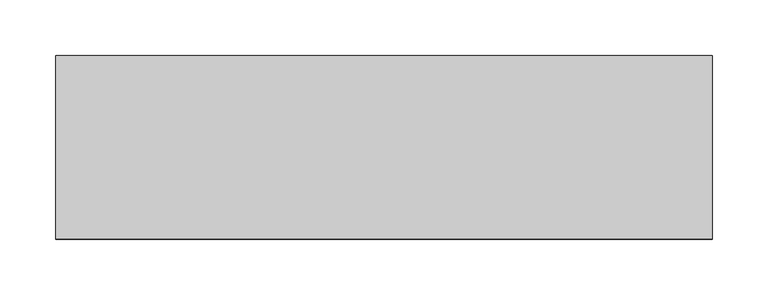
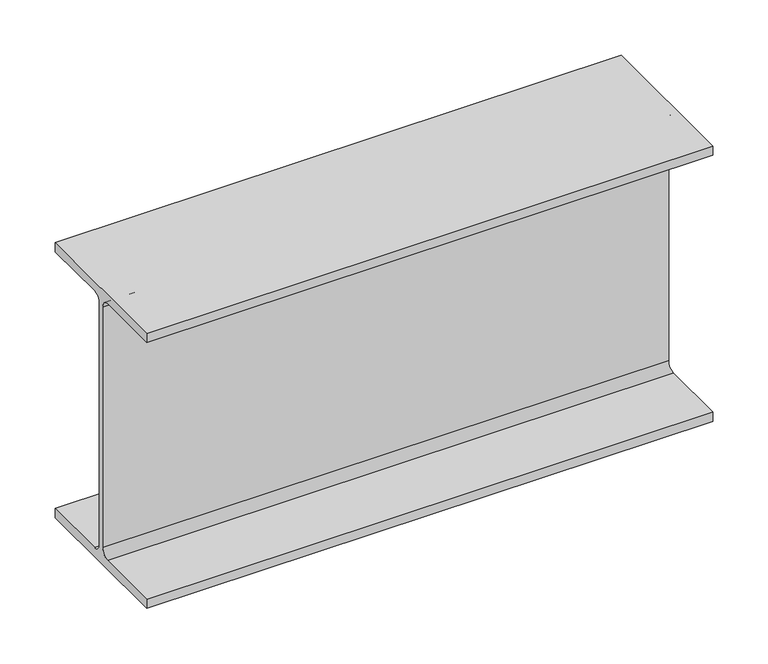
"""IFC4 building model written with IfcOpenShell, lengths in millimetres: beam geometry, Old_Steel Beam_H-KSD3502 : H_SB_ASB_H-300×150x6.5x9."""

import ifcopenshell
import ifcopenshell.guid

model = None  # the IFC model being written
_history = None  # IfcOwnerHistory: only IFC2X3 demands one
_inside = {}  # id of a spatial element -> (the spatial element, [elements in it])
_under = {}  # id of a project, library or spatial element -> (it, [spatial elements below it])
_declared = {}  # id of a project -> (the project, [libraries it declares])
_typed = {}  # id of a type object -> (the type object, [elements of that type])
_made_of = {}  # id of a material, layer set ... -> (it, [elements and type objects made of it])


def new_model(schema):
    """Start an empty IFC model of exactly this schema.

    Asked for "IFC4X3", IfcOpenShell would pick the latest addendum, in which some entities
    have other attributes; the version numbers below select the first issue.
    IFC2X3 requires an IfcOwnerHistory on every rooted entity: one is made here for all.
    """
    global model, _history
    if schema == "IFC4X3":
        model = ifcopenshell.file(schema_version=(4, 3, 0, 0))
    else:
        model = ifcopenshell.file(schema=schema)
    _inside.clear()
    _under.clear()
    _declared.clear()
    _typed.clear()
    _made_of.clear()
    _history = None
    if model.schema == "IFC2X3":
        org = make("IfcOrganization", Name="unknown")
        user = make(
            "IfcPersonAndOrganization",
            ThePerson=make("IfcPerson", FamilyName="unknown"),
            TheOrganization=org,
        )
        app = make(
            "IfcApplication",
            ApplicationDeveloper=org,
            Version="unknown",
            ApplicationFullName="unknown",
            ApplicationIdentifier="unknown",
        )
        _history = make(
            "IfcOwnerHistory",
            OwningUser=user,
            OwningApplication=app,
            ChangeAction="ADDED",
            CreationDate=0,
        )
    return model


def make(cls, **values):
    """One entity of the class cls with the attributes given. An attribute that is None is left unset."""
    return model.create_entity(
        cls, **{name: value for name, value in values.items() if value is not None}
    )


def rooted(cls, **values):
    """An entity with a GlobalId (a new one), such as an element, a storey or a relation."""
    return make(cls, GlobalId=ifcopenshell.guid.new(), OwnerHistory=_history, **values)


def si_unit(unit_type, name, prefix=None):
    """IfcSIUnit, for example si_unit("LENGTHUNIT", "METRE", prefix="MILLI")."""
    return make("IfcSIUnit", UnitType=unit_type, Prefix=prefix, Name=name)


def assignment(units):
    """IfcUnitAssignment: the units of a project."""
    return None if units is None else make("IfcUnitAssignment", Units=units)


def point(xyz):
    """IfcCartesianPoint."""
    return None if xyz is None else make("IfcCartesianPoint", Coordinates=xyz)


def direction(xyz):
    """IfcDirection."""
    return None if xyz is None else make("IfcDirection", DirectionRatios=xyz)


def frame(location, z_axis=None, x_axis=None):
    """IfcAxis2Placement3D, a coordinate frame: its origin and axes. An axis left out is left unset."""
    return make(
        "IfcAxis2Placement3D",
        Location=point(location),
        Axis=direction(z_axis),
        RefDirection=direction(x_axis),
    )


def frame_2d(location, x_axis=None):
    """IfcAxis2Placement2D, a coordinate frame in the plane: its origin and x axis."""
    return make(
        "IfcAxis2Placement2D", Location=point(location), RefDirection=direction(x_axis)
    )


def origin():
    """The frame at (0, 0, 0) with its axes left unset."""
    return frame((0.0, 0.0, 0.0))


def place(relative_to, where):
    """IfcLocalPlacement: puts the frame where relative to a parent placement (None: the world)."""
    return make(
        "IfcLocalPlacement", PlacementRelTo=relative_to, RelativePlacement=where
    )


def context(
    kind, dimensions, precision=None, world=None, true_north=None, identifier=None
):
    """IfcGeometricRepresentationContext, for example the 3D "Model" context."""
    return make(
        "IfcGeometricRepresentationContext",
        ContextIdentifier=identifier,
        ContextType=kind,
        CoordinateSpaceDimension=dimensions,
        Precision=precision,
        WorldCoordinateSystem=world,
        TrueNorth=true_north,
    )


def project(units=None, contexts=None):
    """IfcProject with its units and contexts."""
    return rooted(
        "IfcProject",
        Name="project",
        RepresentationContexts=contexts,
        UnitsInContext=assignment(units),
    )


def spatial(cls, under=None, at=None, **own):
    """A site, building, storey or space (cls), placed at a placement, below another one or the project."""
    s = rooted(cls, ObjectPlacement=at, **own)
    if under is not None:
        _under.setdefault(under.id(), (under, []))[1].append(s)
    return s


def polyline(points):
    """IfcPolyline through the points."""
    return make("IfcPolyline", Points=[point(p) for p in points])


def circle_curve(where, radius):
    """IfcCircle in the frame where."""
    return make("IfcCircle", Position=where, Radius=radius)


def trimmed(basis, trim1, trim2, sense, master):
    """IfcTrimmedCurve: the piece of a basis curve between two trims."""
    return make(
        "IfcTrimmedCurve",
        BasisCurve=basis,
        Trim1=trim1,
        Trim2=trim2,
        SenseAgreement=sense,
        MasterRepresentation=master,
    )


def segment(curve, same_sense, transition):
    """IfcCompositeCurveSegment."""
    return make(
        "IfcCompositeCurveSegment",
        Transition=transition,
        SameSense=same_sense,
        ParentCurve=curve,
    )


def composite_curve(segments, self_intersect=None):
    """IfcCompositeCurve: segments joined end to end."""
    return make("IfcCompositeCurve", Segments=segments, SelfIntersect=self_intersect)


def outline(outer, holes=None, kind="AREA"):
    """IfcArbitraryClosedProfileDef: a profile drawn as a closed curve; with holes, ...WithVoids."""
    if holes is None:
        return make("IfcArbitraryClosedProfileDef", ProfileType=kind, OuterCurve=outer)
    return make(
        "IfcArbitraryProfileDefWithVoids",
        ProfileType=kind,
        OuterCurve=outer,
        InnerCurves=holes,
    )


def extrude(swept, where, along, depth):
    """IfcExtrudedAreaSolid: the profile swept, set in the frame where, extruded along a direction by depth."""
    return make(
        "IfcExtrudedAreaSolid",
        SweptArea=swept,
        Position=where,
        ExtrudedDirection=direction(along),
        Depth=depth,
    )


def shape(context_of_items, identifier, shape_type, items):
    """IfcShapeRepresentation: the items that make up one representation, for example the "Body"."""
    return make(
        "IfcShapeRepresentation",
        ContextOfItems=context_of_items,
        RepresentationIdentifier=identifier,
        RepresentationType=shape_type,
        Items=items,
    )


def source(mapping_origin, context_of_items, identifier, shape_type, items):
    """IfcRepresentationMap: a shape defined once, which mapped items show again and again."""
    return make(
        "IfcRepresentationMap",
        MappingOrigin=mapping_origin,
        MappedRepresentation=shape(context_of_items, identifier, shape_type, items),
    )


def transform(
    local_origin,
    x_axis=None,
    y_axis=None,
    z_axis=None,
    scale=None,
    scale2=None,
    scale3=None,
    uniform=True,
):
    """IfcCartesianTransformationOperator3D, or its non-uniform kind. x_axis, y_axis, z_axis: its Axis1, 2, 3."""
    if uniform:
        return make(
            "IfcCartesianTransformationOperator3D",
            Axis1=direction(x_axis),
            Axis2=direction(y_axis),
            LocalOrigin=point(local_origin),
            Scale=scale,
            Axis3=direction(z_axis),
        )
    return make(
        "IfcCartesianTransformationOperator3DnonUniform",
        Axis1=direction(x_axis),
        Axis2=direction(y_axis),
        LocalOrigin=point(local_origin),
        Scale=scale,
        Axis3=direction(z_axis),
        Scale2=scale2,
        Scale3=scale3,
    )


def mapped(mapping_source, mapping_target):
    """IfcMappedItem: shows the shape of a source again, moved by a transform."""
    return make(
        "IfcMappedItem", MappingSource=mapping_source, MappingTarget=mapping_target
    )


def made_of(thing, what):
    """Note that an element or type object is made of a material, layer set ...; save() writes the relation."""
    if what is not None:
        _made_of.setdefault(what.id(), (what, []))[1].append(thing)
    return thing


def element(
    cls,
    number,
    at=None,
    inside=None,
    cuts=None,
    type_object=None,
    material=None,
    context=None,
    identifier="Body",
    shape_type=None,
    held_by="IfcProductDefinitionShape",
    body=None,
    shapes=None,
    **own,
):
    """One element of the class cls, such as IfcWall. Its Tag is "e" and its number.

    at: its placement. inside: the storey or other place that contains it. cuts: it is an
    opening in that element (IfcRelVoidsElement). A single representation is given by context,
    identifier, shape_type and body (its items); several are given by shapes. held_by: the class
    of the entity that holds the representations. save() writes the other relations.
    """
    e = rooted(cls, Tag="e%d" % number, ObjectPlacement=at, **own)
    if body is not None:
        shapes = [shape(context, identifier, shape_type, body)]
    if shapes is not None:
        e.Representation = make(held_by, Representations=shapes)
    if inside is not None:
        _inside.setdefault(inside.id(), (inside, []))[1].append(e)
    if cuts is not None:
        rooted(
            "IfcRelVoidsElement", RelatingBuildingElement=cuts, RelatedOpeningElement=e
        )
    if type_object is not None:
        _typed.setdefault(type_object.id(), (type_object, []))[1].append(e)
    return made_of(e, material)


def aggregate(whole, parts):
    """IfcRelAggregates: a whole, such as a stair, and the parts it consists of."""
    return rooted("IfcRelAggregates", RelatingObject=whole, RelatedObjects=parts)


def save(model, path):
    """Write the relations noted so far, then the file.

    IfcRelAggregates (storeys below a building ...), IfcRelContainedInSpatialStructure (elements
    in a storey), IfcRelDefinesByType, IfcRelAssociatesMaterial and IfcRelDeclares: one each for
    every whole, place, type object, material and project.
    """
    for whole, parts in _under.values():
        aggregate(whole, parts)
    for where, things in _inside.values():
        rooted(
            "IfcRelContainedInSpatialStructure",
            RelatedElements=things,
            RelatingStructure=where,
        )
    for kind, things in _typed.values():
        rooted("IfcRelDefinesByType", RelatedObjects=things, RelatingType=kind)
    for what, things in _made_of.values():
        rooted("IfcRelAssociatesMaterial", RelatedObjects=things, RelatingMaterial=what)
    for by, libraries in _declared.values():
        rooted("IfcRelDeclares", RelatingContext=by, RelatedDefinitions=libraries)
    model.write(path)


def beam_5c238520(model_context):
    return source(origin(), model_context, "Body", "SweptSolid", [
        extrude(outline(composite_curve([segment(polyline([(82.5, -141.5), (82.5, -151.7), (-82.5, -151.7), (-82.5, -141.5), (-11.9, -141.5)]), True, "CONTINUOUS"), segment(trimmed(circle_curve(frame_2d((-11.9, -132.6)), 8.9), [point((-11.9, -141.5))], [point((-3.0, -132.6))], True, "CARTESIAN"), True, "CONTINUOUS"), segment(polyline([(-3.0, -132.6), (-3.0, 132.6)]), True, "CONTINUOUS"), segment(trimmed(circle_curve(frame_2d((-11.9, 132.6)), 8.9), [point((-3.0, 132.6))], [point((-11.9, 141.5))], True, "CARTESIAN"), True, "CONTINUOUS"), segment(polyline([(-11.9, 141.5), (-82.5, 141.5), (-82.5, 151.7), (82.5, 151.7), (82.5, 141.5), (11.9, 141.5)]), True, "CONTINUOUS"), segment(trimmed(circle_curve(frame_2d((11.9, 132.6)), 8.9), [point((11.9, 141.5))], [point((3.0, 132.6))], True, "CARTESIAN"), True, "CONTINUOUS"), segment(polyline([(3.0, 132.6), (3.0, -132.6)]), True, "CONTINUOUS"), segment(trimmed(circle_curve(frame_2d((11.9, -132.6)), 8.9), [point((3.0, -132.6))], [point((11.9, -141.5))], True, "CARTESIAN"), True, "CONTINUOUS"), segment(polyline([(11.9, -141.5), (82.5, -141.5)]), True, "CONTINUOUS")], self_intersect=False)), frame((-282.3, 0.0, 0.0), z_axis=(1.0, 0.0, 0.0), x_axis=(0.0, 1.0, 0.0)), (0.0, 0.0, 1.0), 589.6),
    ])


if __name__ == "__main__":
    model = new_model("IFC4")
    model_context = context("Model", 3, world=origin())
    ifc_project = project(units=[si_unit("LENGTHUNIT", "METRE", prefix="MILLI")], contexts=[model_context])
    site = spatial("IfcSite", under=ifc_project)
    building = spatial("IfcBuilding", under=site)
    placement = place(None, origin())
    beam_shape = beam_5c238520(model_context)
    element("IfcBeam", 1, ObjectType="Old_Steel Beam_H-KSD3502 : H_SB_ASB_H-300×150x6.5x9", at=placement, inside=building, context=model_context, shape_type="MappedRepresentation", body=[
        mapped(beam_shape, transform((0.0, 0.0, 0.0), x_axis=(1.0, 0.0, 0.0), y_axis=(0.0, 1.0, 0.0), z_axis=(0.0, 0.0, 1.0))),
    ])
    save(model, "model.ifc")

# Revit data of these elements
# Type "Old_Steel Beam_H-KSD3502 : H_SB_ASB_H-300×150x6.5x9"
#   Width = 15.0 cm
#   Web Thickness = 0.65 cm
#   Web Fillet = 1.3 cm
#   Warping Constant = 107174.0 cm⁶
#   Torsional Moment of Inertia = 9.9539 cm⁴
#   Torsional Modulus = 1.0 cm³
#   Section Area = 46.78 cm²
#   Plastic Modulus weak axis = 105.0 cm³
#   Plastic Modulus strong axis = 542.0 cm³
#   Perimeter = 1.17 m²/m
#   Nominal Weight = 36.70 kgf/m
#   Moment of Inertia weak axis = 508.00 cm⁴
#   Moment of Inertia strong axis = 7210.00 cm⁴
#   Height = 30.0 cm
#   Flange Thickness = 0.9 cm
#   Elastic Modulus weak axis = 67.7 cm³
#   Elastic Modulus strong axis = 481.0 cm³
#   Centroid Vertical = 15.0 cm
#   Centroid Horizontal = 7.5 cm
#   Length [instance default] = 1.5240 m
#   Structural Material [instance default] = Steel, 45-345
#   Assembly Code = ""
# Element 1 (IfcBeam, "Old_Steel Beam_H-KSD3502 : H_SB_ASB_H-300×150x6.5x9")
#   Structural Material = none
# Materials
#   "Steel, 45-345": class "Metal", colour RGB 189 187 185, transparency 0, Description = "Steel 345 MPa", Cost = 0
